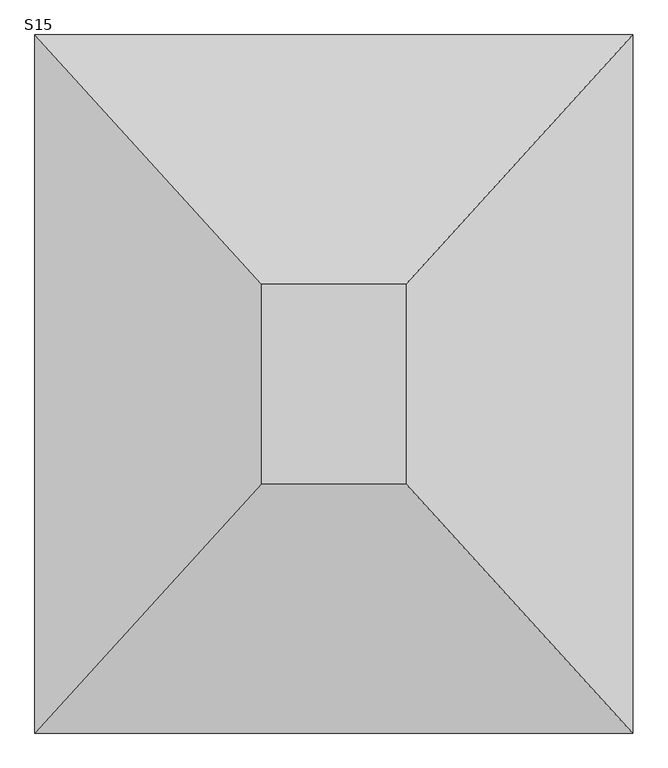
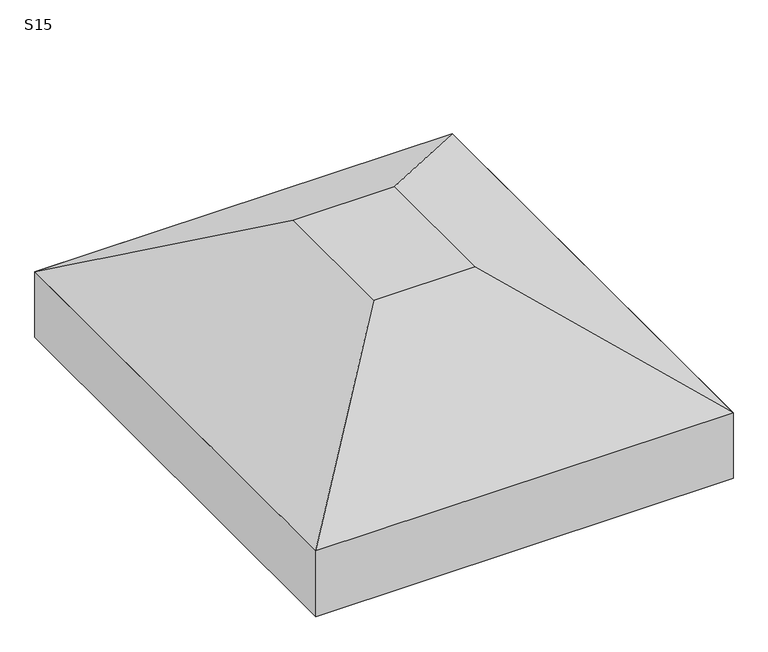
"""IFC4 building model written with IfcOpenShell, lengths in millimetres: fastener geometry, TQS - Sapata : S15."""

import ifcopenshell
import ifcopenshell.guid

model = None  # the IFC model being written
_history = None  # IfcOwnerHistory: only IFC2X3 demands one
_inside = {}  # id of a spatial element -> (the spatial element, [elements in it])
_under = {}  # id of a project, library or spatial element -> (it, [spatial elements below it])
_declared = {}  # id of a project -> (the project, [libraries it declares])
_typed = {}  # id of a type object -> (the type object, [elements of that type])
_made_of = {}  # id of a material, layer set ... -> (it, [elements and type objects made of it])


def new_model(schema):
    """Start an empty IFC model of exactly this schema.

    Asked for "IFC4X3", IfcOpenShell would pick the latest addendum, in which some entities
    have other attributes; the version numbers below select the first issue.
    IFC2X3 requires an IfcOwnerHistory on every rooted entity: one is made here for all.
    """
    global model, _history
    if schema == "IFC4X3":
        model = ifcopenshell.file(schema_version=(4, 3, 0, 0))
    else:
        model = ifcopenshell.file(schema=schema)
    _inside.clear()
    _under.clear()
    _declared.clear()
    _typed.clear()
    _made_of.clear()
    _history = None
    if model.schema == "IFC2X3":
        org = make("IfcOrganization", Name="unknown")
        user = make(
            "IfcPersonAndOrganization",
            ThePerson=make("IfcPerson", FamilyName="unknown"),
            TheOrganization=org,
        )
        app = make(
            "IfcApplication",
            ApplicationDeveloper=org,
            Version="unknown",
            ApplicationFullName="unknown",
            ApplicationIdentifier="unknown",
        )
        _history = make(
            "IfcOwnerHistory",
            OwningUser=user,
            OwningApplication=app,
            ChangeAction="ADDED",
            CreationDate=0,
        )
    return model


def make(cls, **values):
    """One entity of the class cls with the attributes given. An attribute that is None is left unset."""
    return model.create_entity(
        cls, **{name: value for name, value in values.items() if value is not None}
    )


def rooted(cls, **values):
    """An entity with a GlobalId (a new one), such as an element, a storey or a relation."""
    return make(cls, GlobalId=ifcopenshell.guid.new(), OwnerHistory=_history, **values)


def si_unit(unit_type, name, prefix=None):
    """IfcSIUnit, for example si_unit("LENGTHUNIT", "METRE", prefix="MILLI")."""
    return make("IfcSIUnit", UnitType=unit_type, Prefix=prefix, Name=name)


def assignment(units):
    """IfcUnitAssignment: the units of a project."""
    return None if units is None else make("IfcUnitAssignment", Units=units)


def point(xyz):
    """IfcCartesianPoint."""
    return None if xyz is None else make("IfcCartesianPoint", Coordinates=xyz)


def direction(xyz):
    """IfcDirection."""
    return None if xyz is None else make("IfcDirection", DirectionRatios=xyz)


def frame(location, z_axis=None, x_axis=None):
    """IfcAxis2Placement3D, a coordinate frame: its origin and axes. An axis left out is left unset."""
    return make(
        "IfcAxis2Placement3D",
        Location=point(location),
        Axis=direction(z_axis),
        RefDirection=direction(x_axis),
    )


def origin():
    """The frame at (0, 0, 0) with its axes left unset."""
    return frame((0.0, 0.0, 0.0))


def place(relative_to, where):
    """IfcLocalPlacement: puts the frame where relative to a parent placement (None: the world)."""
    return make(
        "IfcLocalPlacement", PlacementRelTo=relative_to, RelativePlacement=where
    )


def context(
    kind, dimensions, precision=None, world=None, true_north=None, identifier=None
):
    """IfcGeometricRepresentationContext, for example the 3D "Model" context."""
    return make(
        "IfcGeometricRepresentationContext",
        ContextIdentifier=identifier,
        ContextType=kind,
        CoordinateSpaceDimension=dimensions,
        Precision=precision,
        WorldCoordinateSystem=world,
        TrueNorth=true_north,
    )


def project(units=None, contexts=None):
    """IfcProject with its units and contexts."""
    return rooted(
        "IfcProject",
        Name="project",
        RepresentationContexts=contexts,
        UnitsInContext=assignment(units),
    )


def spatial(cls, under=None, at=None, **own):
    """A site, building, storey or space (cls), placed at a placement, below another one or the project."""
    s = rooted(cls, ObjectPlacement=at, **own)
    if under is not None:
        _under.setdefault(under.id(), (under, []))[1].append(s)
    return s


def polyline(points):
    """IfcPolyline through the points."""
    return make("IfcPolyline", Points=[point(p) for p in points])


def outline(outer, holes=None, kind="AREA"):
    """IfcArbitraryClosedProfileDef: a profile drawn as a closed curve; with holes, ...WithVoids."""
    if holes is None:
        return make("IfcArbitraryClosedProfileDef", ProfileType=kind, OuterCurve=outer)
    return make(
        "IfcArbitraryProfileDefWithVoids",
        ProfileType=kind,
        OuterCurve=outer,
        InnerCurves=holes,
    )


def extrude(swept, where, along, depth):
    """IfcExtrudedAreaSolid: the profile swept, set in the frame where, extruded along a direction by depth."""
    return make(
        "IfcExtrudedAreaSolid",
        SweptArea=swept,
        Position=where,
        ExtrudedDirection=direction(along),
        Depth=depth,
    )


def faces_of(points, faces, orient=None, outer=None):
    """IfcFace entities. A face is a list of loops; a loop is a list of indices into points, from 0.

    orient and outer hold one flag for each loop. By default every Orientation is true, the
    first loop of a face is its IfcFaceOuterBound and the others are IfcFaceBound.
    """
    made = []
    for i, loops in enumerate(faces):
        bounds = []
        for j, loop in enumerate(loops):
            is_outer = j == 0 if outer is None else outer[i][j]
            bounds.append(
                make(
                    "IfcFaceOuterBound" if is_outer else "IfcFaceBound",
                    Bound=make("IfcPolyLoop", Polygon=[points[k] for k in loop]),
                    Orientation=True if orient is None else orient[i][j],
                )
            )
        made.append(make("IfcFace", Bounds=bounds))
    return made


def faceted_brep(points, faces, orient=None, outer=None, voids=None):
    """IfcFacetedBrep: a solid bounded by flat faces; with voids (closed shells), ...WithVoids."""
    shared = [point(p) for p in points]
    hull = make("IfcClosedShell", CfsFaces=faces_of(shared, faces, orient, outer))
    if voids is None:
        return make("IfcFacetedBrep", Outer=hull)
    return make(
        "IfcFacetedBrepWithVoids",
        Outer=hull,
        Voids=[
            make(cls, CfsFaces=faces_of(shared, fs, o, b)) for cls, fs, o, b in voids
        ],
    )


def shape(context_of_items, identifier, shape_type, items):
    """IfcShapeRepresentation: the items that make up one representation, for example the "Body"."""
    return make(
        "IfcShapeRepresentation",
        ContextOfItems=context_of_items,
        RepresentationIdentifier=identifier,
        RepresentationType=shape_type,
        Items=items,
    )


def source(mapping_origin, context_of_items, identifier, shape_type, items):
    """IfcRepresentationMap: a shape defined once, which mapped items show again and again."""
    return make(
        "IfcRepresentationMap",
        MappingOrigin=mapping_origin,
        MappedRepresentation=shape(context_of_items, identifier, shape_type, items),
    )


def transform(
    local_origin,
    x_axis=None,
    y_axis=None,
    z_axis=None,
    scale=None,
    scale2=None,
    scale3=None,
    uniform=True,
):
    """IfcCartesianTransformationOperator3D, or its non-uniform kind. x_axis, y_axis, z_axis: its Axis1, 2, 3."""
    if uniform:
        return make(
            "IfcCartesianTransformationOperator3D",
            Axis1=direction(x_axis),
            Axis2=direction(y_axis),
            LocalOrigin=point(local_origin),
            Scale=scale,
            Axis3=direction(z_axis),
        )
    return make(
        "IfcCartesianTransformationOperator3DnonUniform",
        Axis1=direction(x_axis),
        Axis2=direction(y_axis),
        LocalOrigin=point(local_origin),
        Scale=scale,
        Axis3=direction(z_axis),
        Scale2=scale2,
        Scale3=scale3,
    )


def mapped(mapping_source, mapping_target):
    """IfcMappedItem: shows the shape of a source again, moved by a transform."""
    return make(
        "IfcMappedItem", MappingSource=mapping_source, MappingTarget=mapping_target
    )


def made_of(thing, what):
    """Note that an element or type object is made of a material, layer set ...; save() writes the relation."""
    if what is not None:
        _made_of.setdefault(what.id(), (what, []))[1].append(thing)
    return thing


def element(
    cls,
    number,
    at=None,
    inside=None,
    cuts=None,
    type_object=None,
    material=None,
    context=None,
    identifier="Body",
    shape_type=None,
    held_by="IfcProductDefinitionShape",
    body=None,
    shapes=None,
    **own,
):
    """One element of the class cls, such as IfcWall. Its Tag is "e" and its number.

    at: its placement. inside: the storey or other place that contains it. cuts: it is an
    opening in that element (IfcRelVoidsElement). A single representation is given by context,
    identifier, shape_type and body (its items); several are given by shapes. held_by: the class
    of the entity that holds the representations. save() writes the other relations.
    """
    e = rooted(cls, Tag="e%d" % number, ObjectPlacement=at, **own)
    if body is not None:
        shapes = [shape(context, identifier, shape_type, body)]
    if shapes is not None:
        e.Representation = make(held_by, Representations=shapes)
    if inside is not None:
        _inside.setdefault(inside.id(), (inside, []))[1].append(e)
    if cuts is not None:
        rooted(
            "IfcRelVoidsElement", RelatingBuildingElement=cuts, RelatedOpeningElement=e
        )
    if type_object is not None:
        _typed.setdefault(type_object.id(), (type_object, []))[1].append(e)
    return made_of(e, material)


def aggregate(whole, parts):
    """IfcRelAggregates: a whole, such as a stair, and the parts it consists of."""
    return rooted("IfcRelAggregates", RelatingObject=whole, RelatedObjects=parts)


def save(model, path):
    """Write the relations noted so far, then the file.

    IfcRelAggregates (storeys below a building ...), IfcRelContainedInSpatialStructure (elements
    in a storey), IfcRelDefinesByType, IfcRelAssociatesMaterial and IfcRelDeclares: one each for
    every whole, place, type object, material and project.
    """
    for whole, parts in _under.values():
        aggregate(whole, parts)
    for where, things in _inside.values():
        rooted(
            "IfcRelContainedInSpatialStructure",
            RelatedElements=things,
            RelatingStructure=where,
        )
    for kind, things in _typed.values():
        rooted("IfcRelDefinesByType", RelatedObjects=things, RelatingType=kind)
    for what, things in _made_of.values():
        rooted("IfcRelAssociatesMaterial", RelatedObjects=things, RelatingMaterial=what)
    for by, libraries in _declared.values():
        rooted("IfcRelDeclares", RelatingContext=by, RelatedDefinitions=libraries)
    model.write(path)


def s15_bbe72304(model_context):
    return source(origin(), model_context, "Body", "SolidModel", [
        faceted_brep([(-55.0, 0.0, 0.0), (-345.0, 0.0, 0.0), (-345.0, -400.0, 0.0), (-55.0, -400.0, 0.0), (400.0, 500.0, -300.0), (400.0, -900.0, -300.0), (-800.0, -900.0, -300.0), (-800.0, 500.0, -300.0)], [[[0, 1, 2, 3]], [[4, 5, 6, 7]], [[4, 7, 1, 0]], [[7, 6, 2, 1]], [[6, 5, 3, 2]], [[5, 4, 0, 3]]]),
        extrude(outline(polyline([(400.0, 500.0), (400.0, -900.0), (-800.0, -900.0), (-800.0, 500.0), (400.0, 500.0)])), frame((0.0, 0.0, -500.0), z_axis=(0.0, 0.0, 1.0), x_axis=(1.0, 0.0, 0.0)), (0.0, 0.0, 1.0), 200.0),
    ])


if __name__ == "__main__":
    model = new_model("IFC4")
    model_context = context("Model", 3, world=origin())
    ifc_project = project(units=[si_unit("LENGTHUNIT", "METRE", prefix="MILLI")], contexts=[model_context])
    site = spatial("IfcSite", under=ifc_project)
    building = spatial("IfcBuilding", under=site)
    placement = place(None, origin())
    s15_shape = s15_bbe72304(model_context)
    element("IfcFastener", 1, ObjectType="TQS - Sapata : S15", at=placement, inside=building, context=model_context, shape_type="MappedRepresentation", body=[
        mapped(s15_shape, transform((0.0, 0.0, 0.0), x_axis=(1.0, 0.0, 0.0), y_axis=(0.0, 1.0, 0.0), z_axis=(0.0, 0.0, 1.0))),
    ])
    save(model, "model.ifc")

# Revit data of these elements
# Type "TQS - Sapata : S15"
#   TY = 0.40 m
#   TX = 0.29 m
#   HS = 0.50 m
#   H0 = 0.20 m
#   EXCYABS = 0.70 m
#   EXCY = 0.00 m
#   EXCXABS = 0.60 m
#   EXCX = 0.00 m
#   DIMY = 1.40 m
#   DIMX = 1.20 m
#   Material estrutural = Concreto - Concreto concretado no local
#   Width = 0
#   Length = 0
# Element 1 (IfcFastener, "TQS - Sapata : S15")
#   Materials on its faces: "Concreto - Concreto concretado no local"
# Materials
#   "Concreto - Concreto concretado no local": class "Concreto", colour RGB 192 192 192, transparency 0
